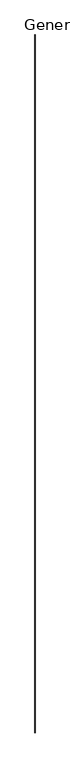
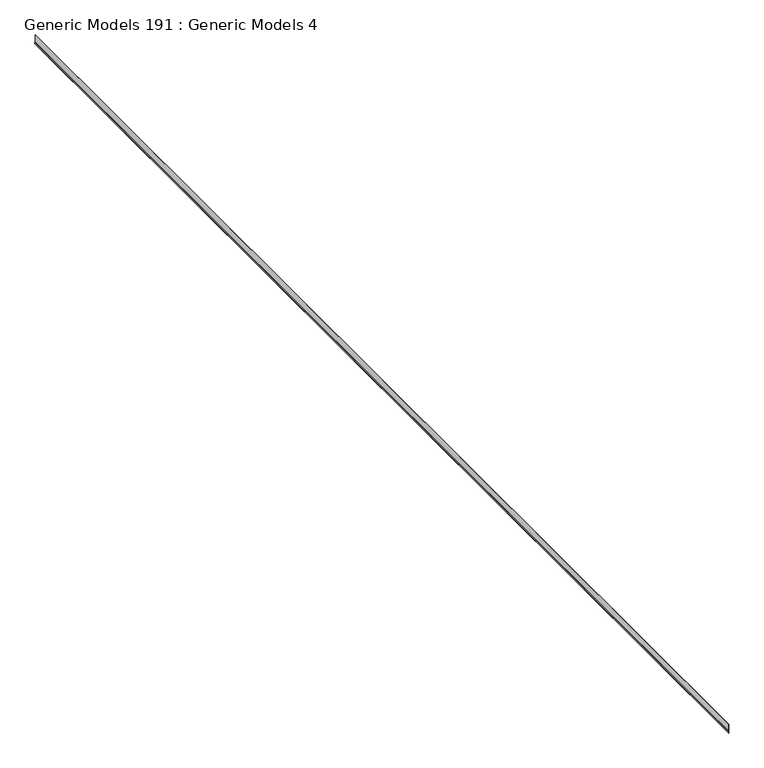
"""IFC4 building model written with IfcOpenShell, lengths in millimetres: proxy geometry, Generic Models 191 : Generic Models 4."""

from ifc_helpers import new_model, si_unit, frame, origin, place, context, project, spatial, polyline, outline, extrude, source, transform, mapped, element, save


def generic_models_191_generic_models_4_1e874bbe(model_context):
    return source(origin(), model_context, "Body", "SweptSolid", [
        extrude(outline(polyline([(126222.1824536, -6614.3104571), (126341.4241678, -6614.3104571), (126341.4241678, -6615.1042071), (126222.3224132, -6615.1042071), (126211.2286669, -6619.1420006), (126196.1749044, -6619.1420006), (126196.1749044, -6618.3482506), (126211.0887074, -6618.3482506), (126222.1824536, -6614.3104571)])), frame((0.0, -6864.9230338, 0.0), z_axis=(0.0, 1.0, 0.0), x_axis=(0.0, 0.0, 1.0)), (0.0, 0.0, 1.0), 18643.6),
    ])


if __name__ == "__main__":
    model = new_model("IFC4")
    model_context = context("Model", 3, world=origin())
    ifc_project = project(units=[si_unit("LENGTHUNIT", "METRE", prefix="MILLI")], contexts=[model_context])
    site = spatial("IfcSite", under=ifc_project)
    building = spatial("IfcBuilding", under=site)
    placement = place(None, origin())
    generic_models_191_generic_models_4_shape = generic_models_191_generic_models_4_1e874bbe(model_context)
    element("IfcBuildingElementProxy", 1, Name="Generic Models 191 : Generic Models 4", ObjectType="Generic Models 191 : Generic Models 4", at=placement, inside=building, context=model_context, shape_type="MappedRepresentation", body=[
        mapped(generic_models_191_generic_models_4_shape, transform((0.0, 0.0, 0.0), x_axis=(1.0, 0.0, 0.0), y_axis=(0.0, 1.0, 0.0), z_axis=(0.0, 0.0, 1.0))),
    ])
    save(model, "model.ifc")

# Revit data of these elements
# Element 1 (IfcBuildingElementProxy, "Generic Models 191 : Generic Models 4")
#   Materials on its faces: "_(2) LAYERS NO. 30 ASTM D226 ASPHALT SATURATED ORGANIC FELT"
# Materials
#   "_(2) LAYERS NO. 30 ASTM D226 ASPHALT SATURATED ORGANIC FELT": class "Generic", colour RGB 67 154 161, transparency 0, Cost = 0
